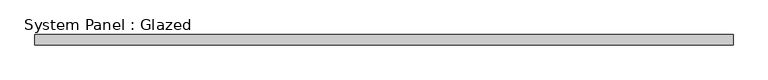
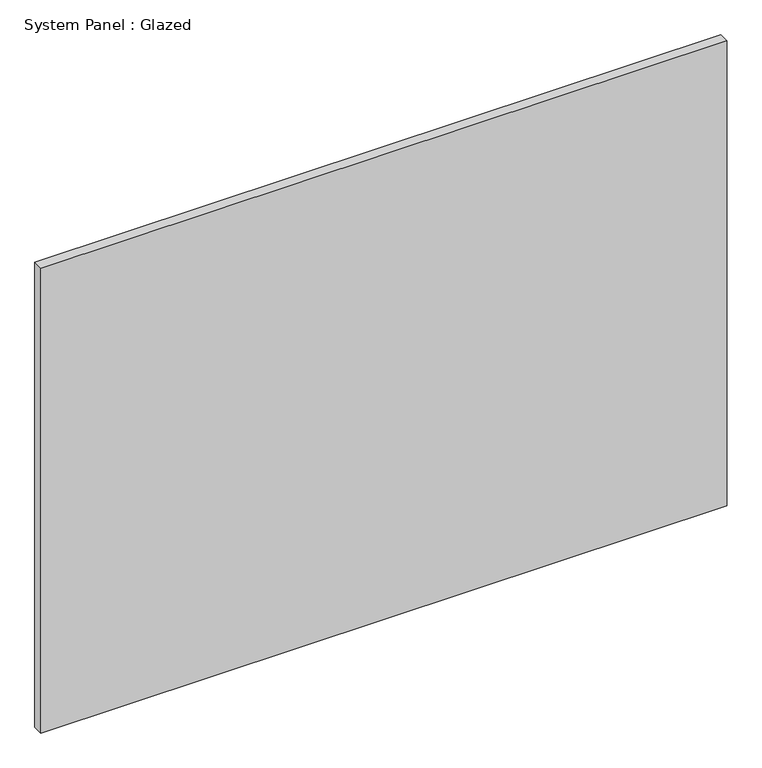
"""IFC4 building model written with IfcOpenShell, lengths in millimetres: plate geometry, System Panel : Glazed."""

from ifc_helpers import new_model, si_unit, origin, origin_with_axes, place, context, project, spatial, polyline, outline, extrude, source, transform, mapped, element, save


def system_panel_glazed_290af845(model_context):
    return source(origin(), model_context, "Body", "SweptSolid", [
        extrude(outline(polyline([(837.5, 24.5), (-837.5, 24.5), (-837.5, 49.5), (837.5, 49.5), (837.5, 24.5)])), origin_with_axes(), (0.0, 0.0, 1.0), 1200.0),
    ])


if __name__ == "__main__":
    model = new_model("IFC4")
    model_context = context("Model", 3, world=origin())
    ifc_project = project(units=[si_unit("LENGTHUNIT", "METRE", prefix="MILLI")], contexts=[model_context])
    site = spatial("IfcSite", under=ifc_project)
    building = spatial("IfcBuilding", under=site)
    placement = place(None, origin())
    system_panel_glazed_shape = system_panel_glazed_290af845(model_context)
    element("IfcPlate", 1, ObjectType="System Panel : Glazed", at=placement, inside=building, context=model_context, shape_type="MappedRepresentation", body=[
        mapped(system_panel_glazed_shape, transform((0.0, 0.0, 0.0), x_axis=(1.0, 0.0, 0.0), y_axis=(0.0, 1.0, 0.0), z_axis=(0.0, 0.0, 1.0))),
    ])
    save(model, "model.ifc")

# Revit data of these elements
# Element 1 (IfcPlate, "System Panel : Glazed")
#   Materials on its faces: "Glass"
# Materials
#   "Glass": class "Glass", colour RGB 218 227 224, transparency 0.85, Description = "Soda Lime Glass", Cost = 0
